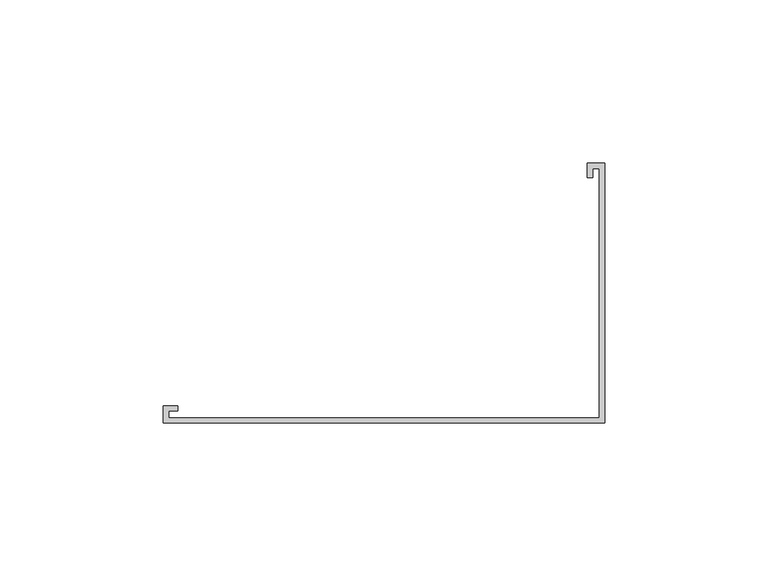
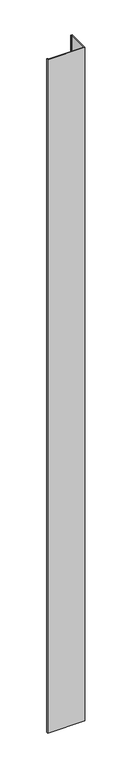
"""IFC4 building model written with IfcOpenShell, lengths in millimetres: proxy geometry, Generic Models 2:Generic Models 2:310765:Generic Models 2:310765 : Generic Models 2:Generic Models 2:310765:54 : Generic Models 2:Generic Models 2:310765:Generic Models 2:310765 : Generic Models 2:Generic Models 2:310765:300385."""

from ifc_helpers import new_model, si_unit, frame, origin, place, context, project, spatial, polyline, outline, extrude, source, transform, mapped, element, save


def generic_models_8a1801b6(model_context):
    return source(origin(), model_context, "Body", "SweptSolid", [
        extrude(outline(polyline([(667604.2742598, -568167.1930453), (667609.5456314, -568167.1930453), (667609.5456314, -568246.7052305), (667474.5588141, -568246.7052305), (667474.5588141, -568241.4338589), (667478.9461407, -568241.4338589), (667478.9461407, -568243.0213589), (667476.1463141, -568243.0213589), (667476.1463141, -568245.1177305), (667607.9581314, -568245.1177305), (667607.9581314, -568168.7805453), (667605.8617598, -568168.7805453), (667605.8617598, -568171.5803719), (667604.2742598, -568171.5803719), (667604.2742598, -568167.1930453)])), frame((0.0, 0.0, 6187.7226497), z_axis=(0.0, 0.0, 1.0), x_axis=(1.0, 0.0, 0.0)), (0.0, 0.0, 1.0), 2588.1508001),
    ])


if __name__ == "__main__":
    model = new_model("IFC4")
    model_context = context("Model", 3, world=origin())
    ifc_project = project(units=[si_unit("LENGTHUNIT", "METRE", prefix="MILLI")], contexts=[model_context])
    site = spatial("IfcSite", under=ifc_project)
    building = spatial("IfcBuilding", under=site)
    placement = place(None, origin())
    generic_models_shape = generic_models_8a1801b6(model_context)
    element("IfcBuildingElementProxy", 1, Name="Generic Models 2:Generic Models 2:310765:Generic Models 2:310765 : Generic Models 2:Generic Models 2:310765:54 : Generic Models 2:Generic Models 2:310765:Generic Models 2:310765 : Generic Models 2:Generic Models 2:310765:300385", ObjectType="Generic Models 2:Generic Models 2:310765:Generic Models 2:310765 : Generic Models 2:Generic Models 2:310765:54 : Generic Models 2:Generic Models 2:310765:Generic Models 2:310765 : Generic Models 2:Generic Models 2:310765:300385", at=placement, inside=building, context=model_context, shape_type="MappedRepresentation", body=[
        mapped(generic_models_shape, transform((0.0, 0.0, 0.0), x_axis=(1.0, 0.0, 0.0), y_axis=(0.0, 1.0, 0.0), z_axis=(0.0, 0.0, 1.0))),
    ])
    save(model, "model.ifc")

# Revit data of these elements
# Type "Generic Models 2:Generic Models 2:310765:Generic Models 2:310765 : Generic Models 2:Generic Models 2:310765:54 : Generic Models 2:Generic Models 2:310765:Generic Models 2:310765 : Generic Models 2:Generic Models 2:310765:300385"
#   NameOverride = "Generic Models 2:Generic Models 2:310765:Generic Models 2:310765 : Generic Models 2:Generic Models 2:310765:300385"
#   ObjectTypeOverride = "Generic Models 2:310765 : Generic Models 2:Generic Models 2:310765"
#   Reference = "Generic Models 2"
#   Tag = "300385"
# Element 1 (IfcBuildingElementProxy, "Generic Models 2:Generic Models 2:310765:Generic Models 2:310765 : Generic Models 2:Generic Models 2:310765:54 : Generic Models 2:Generic Models 2:310765:Generic Models 2:310765 : Generic Models 2:Generic Models 2:310765:300385")
#   Materials on its faces: "BRAKE METAL CLOSURE TRIM"
# Materials
#   "BRAKE METAL CLOSURE TRIM": class "Unassigned", colour RGB 182 182 182, transparency 0, Cost = 0
